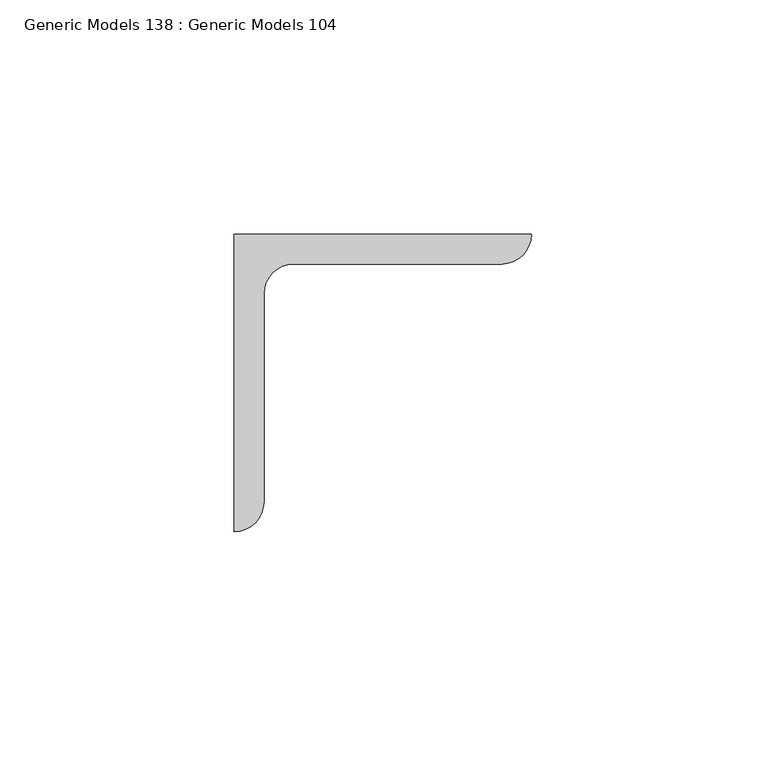
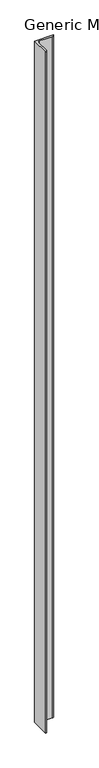
"""IFC4 building model written with IfcOpenShell, lengths in millimetres: proxy geometry, Generic Models 138 : Generic Models 104."""

from ifc_helpers import new_model, si_unit, point, frame, frame_2d, origin, place, context, project, spatial, polyline, circle_curve, trimmed, segment, composite_curve, outline, extrude, source, transform, mapped, element, save


def generic_models_138_generic_models_104_8be79013(model_context):
    return source(origin(), model_context, "Body", "SweptSolid", [
        extrude(outline(composite_curve([segment(polyline([(30226.3140778, 41071.1196612), (30289.8140778, 41071.1196612)]), True, "CONTINUOUS"), segment(trimmed(circle_curve(frame_2d((30283.4640778, 41071.1196612)), 6.35), [point((30289.8140778, 41071.1196612))], [point((30283.4640778, 41064.7696612))], False, "CARTESIAN"), True, "CONTINUOUS"), segment(polyline([(30283.4640778, 41064.7696612), (30239.0140778, 41064.7696612)]), True, "CONTINUOUS"), segment(trimmed(circle_curve(frame_2d((30239.0140778, 41058.4196612)), 6.35), [point((30239.0140778, 41064.7696612))], [point((30232.6640778, 41058.4196612))], True, "CARTESIAN"), True, "CONTINUOUS"), segment(polyline([(30232.6640778, 41058.4196612), (30232.6640778, 41013.9696612)]), True, "CONTINUOUS"), segment(trimmed(circle_curve(frame_2d((30226.3140778, 41013.9696612)), 6.35), [point((30232.6640778, 41013.9696612))], [point((30226.3140778, 41007.6196612))], False, "CARTESIAN"), True, "CONTINUOUS"), segment(polyline([(30226.3140778, 41007.6196612), (30226.3140778, 41071.1196612)]), True, "CONTINUOUS")], self_intersect=False)), frame((0.0, 0.0, 266407.9), z_axis=(0.0, 0.0, 1.0), x_axis=(1.0, 0.0, 0.0)), (0.0, 0.0, 1.0), 2432.1044757),
    ])


if __name__ == "__main__":
    model = new_model("IFC4")
    model_context = context("Model", 3, world=origin())
    ifc_project = project(units=[si_unit("LENGTHUNIT", "METRE", prefix="MILLI")], contexts=[model_context])
    site = spatial("IfcSite", under=ifc_project)
    building = spatial("IfcBuilding", under=site)
    placement = place(None, origin())
    generic_models_138_generic_models_104_shape = generic_models_138_generic_models_104_8be79013(model_context)
    element("IfcBuildingElementProxy", 1, Name="Generic Models 138 : Generic Models 104", ObjectType="Generic Models 138 : Generic Models 104", at=placement, inside=building, context=model_context, shape_type="MappedRepresentation", body=[
        mapped(generic_models_138_generic_models_104_shape, transform((0.0, 0.0, 0.0), x_axis=(1.0, 0.0, 0.0), y_axis=(0.0, 1.0, 0.0), z_axis=(0.0, 0.0, 1.0))),
    ])
    save(model, "model.ifc")

# Revit data of these elements
# Element 1 (IfcBuildingElementProxy, "Generic Models 138 : Generic Models 104")
#   Materials on its faces: "(2) BACK/BACK GALVANIZED ANGLES (2) L2 1/2 X 2 1/2 X 1/4\")"
# Materials
#   "(2) BACK/BACK GALVANIZED ANGLES (2) L2 1/2 X 2 1/2 X 1/4\")": class "Unassigned", colour RGB 211 211 211, transparency 0, Cost = 0
